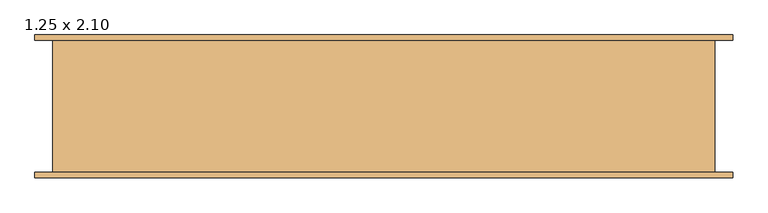
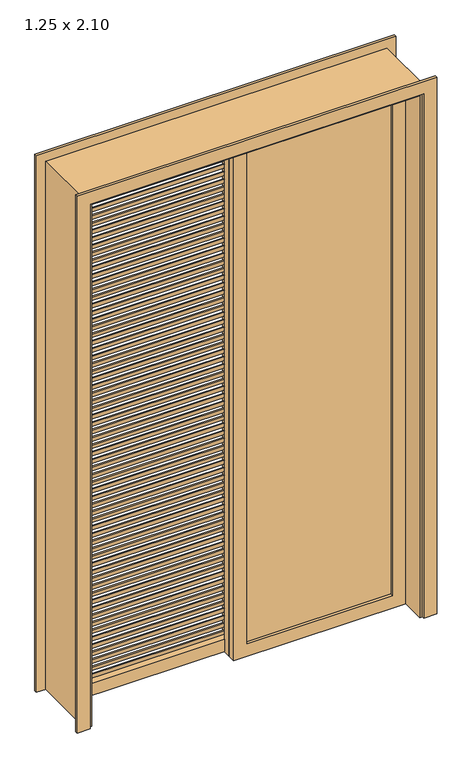
"""IFC4 building model written with IfcOpenShell, lengths in millimetres: door geometry, .CC_ND 300_PORTA DE CORRER_3 FOLHAS_VENEZIANA_VIDRO_COM EXTENSÃO : 1.25 x 2.10."""

from ifc_helpers import new_model, si_unit, frame, origin, place, context, project, spatial, polyline, outline, extrude, source, transform, mapped, element, save


def door_1_25_x_2_10_d20a60c6(model_context):
    return source(origin(), model_context, "Body", "SweptSolid", [
        extrude(outline(polyline([(575.0, -26.0), (575.0, -34.0), (20.0, -34.0), (20.0, -26.0), (575.0, -26.0)])), frame((0.0, 0.0, 50.0), z_axis=(0.0, 0.0, 1.0), x_axis=(1.0, 0.0, 0.0)), (0.0, 0.0, 1.0), 2000.0),
        extrude(outline(polyline([(2100.0, 625.0), (2100.0, -30.0), (0.0, -30.0), (0.0, 625.0), (2100.0, 625.0)]), holes=[polyline([(2050.0, 575.0), (50.0, 575.0), (50.0, 20.0), (2050.0, 20.0), (2050.0, 575.0)])]), frame((0.0, -45.0, 0.0), z_axis=(0.0, 1.0, 0.0), x_axis=(0.0, 0.0, 1.0)), (0.0, 0.0, 1.0), 30.0),
        extrude(outline(polyline([(40.0, 1985.2272727), (15.0, 2020.2272727), (20.0, 2020.2272727), (45.0, 1985.2272727), (40.0, 1985.2272727)])), frame((-575.0, 0.0, 0.0), z_axis=(1.0, 0.0, 0.0), x_axis=(0.0, 1.0, 0.0)), (0.0, 0.0, 1.0), 555.0),
        extrude(outline(polyline([(40.0, 1955.4545455), (15.0, 1990.4545455), (20.0, 1990.4545455), (45.0, 1955.4545455), (40.0, 1955.4545455)])), frame((-575.0, 0.0, 0.0), z_axis=(1.0, 0.0, 0.0), x_axis=(0.0, 1.0, 0.0)), (0.0, 0.0, 1.0), 555.0),
        extrude(outline(polyline([(40.0, 1925.6818182), (15.0, 1960.6818182), (20.0, 1960.6818182), (45.0, 1925.6818182), (40.0, 1925.6818182)])), frame((-575.0, 0.0, 0.0), z_axis=(1.0, 0.0, 0.0), x_axis=(0.0, 1.0, 0.0)), (0.0, 0.0, 1.0), 555.0),
        extrude(outline(polyline([(40.0, 1895.9090909), (15.0, 1930.9090909), (20.0, 1930.9090909), (45.0, 1895.9090909), (40.0, 1895.9090909)])), frame((-575.0, 0.0, 0.0), z_axis=(1.0, 0.0, 0.0), x_axis=(0.0, 1.0, 0.0)), (0.0, 0.0, 1.0), 555.0),
        extrude(outline(polyline([(40.0, 1866.1363636), (15.0, 1901.1363636), (20.0, 1901.1363636), (45.0, 1866.1363636), (40.0, 1866.1363636)])), frame((-575.0, 0.0, 0.0), z_axis=(1.0, 0.0, 0.0), x_axis=(0.0, 1.0, 0.0)), (0.0, 0.0, 1.0), 555.0),
        extrude(outline(polyline([(40.0, 1836.3636364), (15.0, 1871.3636364), (20.0, 1871.3636364), (45.0, 1836.3636364), (40.0, 1836.3636364)])), frame((-575.0, 0.0, 0.0), z_axis=(1.0, 0.0, 0.0), x_axis=(0.0, 1.0, 0.0)), (0.0, 0.0, 1.0), 555.0),
        extrude(outline(polyline([(40.0, 1806.5909091), (15.0, 1841.5909091), (20.0, 1841.5909091), (45.0, 1806.5909091), (40.0, 1806.5909091)])), frame((-575.0, 0.0, 0.0), z_axis=(1.0, 0.0, 0.0), x_axis=(0.0, 1.0, 0.0)), (0.0, 0.0, 1.0), 555.0),
        extrude(outline(polyline([(40.0, 1776.8181818), (15.0, 1811.8181818), (20.0, 1811.8181818), (45.0, 1776.8181818), (40.0, 1776.8181818)])), frame((-575.0, 0.0, 0.0), z_axis=(1.0, 0.0, 0.0), x_axis=(0.0, 1.0, 0.0)), (0.0, 0.0, 1.0), 555.0),
        extrude(outline(polyline([(40.0, 1747.0454545), (15.0, 1782.0454545), (20.0, 1782.0454545), (45.0, 1747.0454545), (40.0, 1747.0454545)])), frame((-575.0, 0.0, 0.0), z_axis=(1.0, 0.0, 0.0), x_axis=(0.0, 1.0, 0.0)), (0.0, 0.0, 1.0), 555.0),
        extrude(outline(polyline([(40.0, 1717.2727273), (15.0, 1752.2727273), (20.0, 1752.2727273), (45.0, 1717.2727273), (40.0, 1717.2727273)])), frame((-575.0, 0.0, 0.0), z_axis=(1.0, 0.0, 0.0), x_axis=(0.0, 1.0, 0.0)), (0.0, 0.0, 1.0), 555.0),
        extrude(outline(polyline([(40.0, 1687.5), (15.0, 1722.5), (20.0, 1722.5), (45.0, 1687.5), (40.0, 1687.5)])), frame((-575.0, 0.0, 0.0), z_axis=(1.0, 0.0, 0.0), x_axis=(0.0, 1.0, 0.0)), (0.0, 0.0, 1.0), 555.0),
        extrude(outline(polyline([(40.0, 1657.7272727), (15.0, 1692.7272727), (20.0, 1692.7272727), (45.0, 1657.7272727), (40.0, 1657.7272727)])), frame((-575.0, 0.0, 0.0), z_axis=(1.0, 0.0, 0.0), x_axis=(0.0, 1.0, 0.0)), (0.0, 0.0, 1.0), 555.0),
        extrude(outline(polyline([(40.0, 1627.9545455), (15.0, 1662.9545455), (20.0, 1662.9545455), (45.0, 1627.9545455), (40.0, 1627.9545455)])), frame((-575.0, 0.0, 0.0), z_axis=(1.0, 0.0, 0.0), x_axis=(0.0, 1.0, 0.0)), (0.0, 0.0, 1.0), 555.0),
        extrude(outline(polyline([(40.0, 1598.1818182), (15.0, 1633.1818182), (20.0, 1633.1818182), (45.0, 1598.1818182), (40.0, 1598.1818182)])), frame((-575.0, 0.0, 0.0), z_axis=(1.0, 0.0, 0.0), x_axis=(0.0, 1.0, 0.0)), (0.0, 0.0, 1.0), 555.0),
        extrude(outline(polyline([(40.0, 1568.4090909), (15.0, 1603.4090909), (20.0, 1603.4090909), (45.0, 1568.4090909), (40.0, 1568.4090909)])), frame((-575.0, 0.0, 0.0), z_axis=(1.0, 0.0, 0.0), x_axis=(0.0, 1.0, 0.0)), (0.0, 0.0, 1.0), 555.0),
        extrude(outline(polyline([(40.0, 1538.6363636), (15.0, 1573.6363636), (20.0, 1573.6363636), (45.0, 1538.6363636), (40.0, 1538.6363636)])), frame((-575.0, 0.0, 0.0), z_axis=(1.0, 0.0, 0.0), x_axis=(0.0, 1.0, 0.0)), (0.0, 0.0, 1.0), 555.0),
        extrude(outline(polyline([(40.0, 1508.8636364), (15.0, 1543.8636364), (20.0, 1543.8636364), (45.0, 1508.8636364), (40.0, 1508.8636364)])), frame((-575.0, 0.0, 0.0), z_axis=(1.0, 0.0, 0.0), x_axis=(0.0, 1.0, 0.0)), (0.0, 0.0, 1.0), 555.0),
        extrude(outline(polyline([(40.0, 1479.0909091), (15.0, 1514.0909091), (20.0, 1514.0909091), (45.0, 1479.0909091), (40.0, 1479.0909091)])), frame((-575.0, 0.0, 0.0), z_axis=(1.0, 0.0, 0.0), x_axis=(0.0, 1.0, 0.0)), (0.0, 0.0, 1.0), 555.0),
        extrude(outline(polyline([(40.0, 1449.3181818), (15.0, 1484.3181818), (20.0, 1484.3181818), (45.0, 1449.3181818), (40.0, 1449.3181818)])), frame((-575.0, 0.0, 0.0), z_axis=(1.0, 0.0, 0.0), x_axis=(0.0, 1.0, 0.0)), (0.0, 0.0, 1.0), 555.0),
        extrude(outline(polyline([(40.0, 1419.5454545), (15.0, 1454.5454545), (20.0, 1454.5454545), (45.0, 1419.5454545), (40.0, 1419.5454545)])), frame((-575.0, 0.0, 0.0), z_axis=(1.0, 0.0, 0.0), x_axis=(0.0, 1.0, 0.0)), (0.0, 0.0, 1.0), 555.0),
        extrude(outline(polyline([(40.0, 1389.7727273), (15.0, 1424.7727273), (20.0, 1424.7727273), (45.0, 1389.7727273), (40.0, 1389.7727273)])), frame((-575.0, 0.0, 0.0), z_axis=(1.0, 0.0, 0.0), x_axis=(0.0, 1.0, 0.0)), (0.0, 0.0, 1.0), 555.0),
        extrude(outline(polyline([(40.0, 1360.0), (15.0, 1395.0), (20.0, 1395.0), (45.0, 1360.0), (40.0, 1360.0)])), frame((-575.0, 0.0, 0.0), z_axis=(1.0, 0.0, 0.0), x_axis=(0.0, 1.0, 0.0)), (0.0, 0.0, 1.0), 555.0),
        extrude(outline(polyline([(40.0, 1330.2272727), (15.0, 1365.2272727), (20.0, 1365.2272727), (45.0, 1330.2272727), (40.0, 1330.2272727)])), frame((-575.0, 0.0, 0.0), z_axis=(1.0, 0.0, 0.0), x_axis=(0.0, 1.0, 0.0)), (0.0, 0.0, 1.0), 555.0),
        extrude(outline(polyline([(40.0, 1300.4545455), (15.0, 1335.4545455), (20.0, 1335.4545455), (45.0, 1300.4545455), (40.0, 1300.4545455)])), frame((-575.0, 0.0, 0.0), z_axis=(1.0, 0.0, 0.0), x_axis=(0.0, 1.0, 0.0)), (0.0, 0.0, 1.0), 555.0),
        extrude(outline(polyline([(40.0, 1270.6818182), (15.0, 1305.6818182), (20.0, 1305.6818182), (45.0, 1270.6818182), (40.0, 1270.6818182)])), frame((-575.0, 0.0, 0.0), z_axis=(1.0, 0.0, 0.0), x_axis=(0.0, 1.0, 0.0)), (0.0, 0.0, 1.0), 555.0),
        extrude(outline(polyline([(40.0, 1240.9090909), (15.0, 1275.9090909), (20.0, 1275.9090909), (45.0, 1240.9090909), (40.0, 1240.9090909)])), frame((-575.0, 0.0, 0.0), z_axis=(1.0, 0.0, 0.0), x_axis=(0.0, 1.0, 0.0)), (0.0, 0.0, 1.0), 555.0),
        extrude(outline(polyline([(40.0, 1211.1363636), (15.0, 1246.1363636), (20.0, 1246.1363636), (45.0, 1211.1363636), (40.0, 1211.1363636)])), frame((-575.0, 0.0, 0.0), z_axis=(1.0, 0.0, 0.0), x_axis=(0.0, 1.0, 0.0)), (0.0, 0.0, 1.0), 555.0),
        extrude(outline(polyline([(40.0, 1181.3636364), (15.0, 1216.3636364), (20.0, 1216.3636364), (45.0, 1181.3636364), (40.0, 1181.3636364)])), frame((-575.0, 0.0, 0.0), z_axis=(1.0, 0.0, 0.0), x_axis=(0.0, 1.0, 0.0)), (0.0, 0.0, 1.0), 555.0),
        extrude(outline(polyline([(40.0, 1151.5909091), (15.0, 1186.5909091), (20.0, 1186.5909091), (45.0, 1151.5909091), (40.0, 1151.5909091)])), frame((-575.0, 0.0, 0.0), z_axis=(1.0, 0.0, 0.0), x_axis=(0.0, 1.0, 0.0)), (0.0, 0.0, 1.0), 555.0),
        extrude(outline(polyline([(40.0, 1121.8181818), (15.0, 1156.8181818), (20.0, 1156.8181818), (45.0, 1121.8181818), (40.0, 1121.8181818)])), frame((-575.0, 0.0, 0.0), z_axis=(1.0, 0.0, 0.0), x_axis=(0.0, 1.0, 0.0)), (0.0, 0.0, 1.0), 555.0),
        extrude(outline(polyline([(40.0, 1092.0454545), (15.0, 1127.0454545), (20.0, 1127.0454545), (45.0, 1092.0454545), (40.0, 1092.0454545)])), frame((-575.0, 0.0, 0.0), z_axis=(1.0, 0.0, 0.0), x_axis=(0.0, 1.0, 0.0)), (0.0, 0.0, 1.0), 555.0),
        extrude(outline(polyline([(40.0, 1062.2727273), (15.0, 1097.2727273), (20.0, 1097.2727273), (45.0, 1062.2727273), (40.0, 1062.2727273)])), frame((-575.0, 0.0, 0.0), z_axis=(1.0, 0.0, 0.0), x_axis=(0.0, 1.0, 0.0)), (0.0, 0.0, 1.0), 555.0),
        extrude(outline(polyline([(40.0, 1032.5), (15.0, 1067.5), (20.0, 1067.5), (45.0, 1032.5), (40.0, 1032.5)])), frame((-575.0, 0.0, 0.0), z_axis=(1.0, 0.0, 0.0), x_axis=(0.0, 1.0, 0.0)), (0.0, 0.0, 1.0), 555.0),
        extrude(outline(polyline([(40.0, 1002.7272727), (15.0, 1037.7272727), (20.0, 1037.7272727), (45.0, 1002.7272727), (40.0, 1002.7272727)])), frame((-575.0, 0.0, 0.0), z_axis=(1.0, 0.0, 0.0), x_axis=(0.0, 1.0, 0.0)), (0.0, 0.0, 1.0), 555.0),
        extrude(outline(polyline([(40.0, 972.9545455), (15.0, 1007.9545455), (20.0, 1007.9545455), (45.0, 972.9545455), (40.0, 972.9545455)])), frame((-575.0, 0.0, 0.0), z_axis=(1.0, 0.0, 0.0), x_axis=(0.0, 1.0, 0.0)), (0.0, 0.0, 1.0), 555.0),
        extrude(outline(polyline([(40.0, 943.1818182), (15.0, 978.1818182), (20.0, 978.1818182), (45.0, 943.1818182), (40.0, 943.1818182)])), frame((-575.0, 0.0, 0.0), z_axis=(1.0, 0.0, 0.0), x_axis=(0.0, 1.0, 0.0)), (0.0, 0.0, 1.0), 555.0),
        extrude(outline(polyline([(40.0, 913.4090909), (15.0, 948.4090909), (20.0, 948.4090909), (45.0, 913.4090909), (40.0, 913.4090909)])), frame((-575.0, 0.0, 0.0), z_axis=(1.0, 0.0, 0.0), x_axis=(0.0, 1.0, 0.0)), (0.0, 0.0, 1.0), 555.0),
        extrude(outline(polyline([(40.0, 883.6363636), (15.0, 918.6363636), (20.0, 918.6363636), (45.0, 883.6363636), (40.0, 883.6363636)])), frame((-575.0, 0.0, 0.0), z_axis=(1.0, 0.0, 0.0), x_axis=(0.0, 1.0, 0.0)), (0.0, 0.0, 1.0), 555.0),
        extrude(outline(polyline([(40.0, 853.8636364), (15.0, 888.8636364), (20.0, 888.8636364), (45.0, 853.8636364), (40.0, 853.8636364)])), frame((-575.0, 0.0, 0.0), z_axis=(1.0, 0.0, 0.0), x_axis=(0.0, 1.0, 0.0)), (0.0, 0.0, 1.0), 555.0),
        extrude(outline(polyline([(40.0, 824.0909091), (15.0, 859.0909091), (20.0, 859.0909091), (45.0, 824.0909091), (40.0, 824.0909091)])), frame((-575.0, 0.0, 0.0), z_axis=(1.0, 0.0, 0.0), x_axis=(0.0, 1.0, 0.0)), (0.0, 0.0, 1.0), 555.0),
        extrude(outline(polyline([(40.0, 794.3181818), (15.0, 829.3181818), (20.0, 829.3181818), (45.0, 794.3181818), (40.0, 794.3181818)])), frame((-575.0, 0.0, 0.0), z_axis=(1.0, 0.0, 0.0), x_axis=(0.0, 1.0, 0.0)), (0.0, 0.0, 1.0), 555.0),
        extrude(outline(polyline([(40.0, 764.5454545), (15.0, 799.5454545), (20.0, 799.5454545), (45.0, 764.5454545), (40.0, 764.5454545)])), frame((-575.0, 0.0, 0.0), z_axis=(1.0, 0.0, 0.0), x_axis=(0.0, 1.0, 0.0)), (0.0, 0.0, 1.0), 555.0),
        extrude(outline(polyline([(40.0, 734.7727273), (15.0, 769.7727273), (20.0, 769.7727273), (45.0, 734.7727273), (40.0, 734.7727273)])), frame((-575.0, 0.0, 0.0), z_axis=(1.0, 0.0, 0.0), x_axis=(0.0, 1.0, 0.0)), (0.0, 0.0, 1.0), 555.0),
        extrude(outline(polyline([(40.0, 705.0), (15.0, 740.0), (20.0, 740.0), (45.0, 705.0), (40.0, 705.0)])), frame((-575.0, 0.0, 0.0), z_axis=(1.0, 0.0, 0.0), x_axis=(0.0, 1.0, 0.0)), (0.0, 0.0, 1.0), 555.0),
        extrude(outline(polyline([(40.0, 675.2272727), (15.0, 710.2272727), (20.0, 710.2272727), (45.0, 675.2272727), (40.0, 675.2272727)])), frame((-575.0, 0.0, 0.0), z_axis=(1.0, 0.0, 0.0), x_axis=(0.0, 1.0, 0.0)), (0.0, 0.0, 1.0), 555.0),
        extrude(outline(polyline([(40.0, 645.4545455), (15.0, 680.4545455), (20.0, 680.4545455), (45.0, 645.4545455), (40.0, 645.4545455)])), frame((-575.0, 0.0, 0.0), z_axis=(1.0, 0.0, 0.0), x_axis=(0.0, 1.0, 0.0)), (0.0, 0.0, 1.0), 555.0),
        extrude(outline(polyline([(40.0, 615.6818182), (15.0, 650.6818182), (20.0, 650.6818182), (45.0, 615.6818182), (40.0, 615.6818182)])), frame((-575.0, 0.0, 0.0), z_axis=(1.0, 0.0, 0.0), x_axis=(0.0, 1.0, 0.0)), (0.0, 0.0, 1.0), 555.0),
        extrude(outline(polyline([(40.0, 585.9090909), (15.0, 620.9090909), (20.0, 620.9090909), (45.0, 585.9090909), (40.0, 585.9090909)])), frame((-575.0, 0.0, 0.0), z_axis=(1.0, 0.0, 0.0), x_axis=(0.0, 1.0, 0.0)), (0.0, 0.0, 1.0), 555.0),
        extrude(outline(polyline([(40.0, 556.1363636), (15.0, 591.1363636), (20.0, 591.1363636), (45.0, 556.1363636), (40.0, 556.1363636)])), frame((-575.0, 0.0, 0.0), z_axis=(1.0, 0.0, 0.0), x_axis=(0.0, 1.0, 0.0)), (0.0, 0.0, 1.0), 555.0),
        extrude(outline(polyline([(40.0, 526.3636364), (15.0, 561.3636364), (20.0, 561.3636364), (45.0, 526.3636364), (40.0, 526.3636364)])), frame((-575.0, 0.0, 0.0), z_axis=(1.0, 0.0, 0.0), x_axis=(0.0, 1.0, 0.0)), (0.0, 0.0, 1.0), 555.0),
        extrude(outline(polyline([(40.0, 496.5909091), (15.0, 531.5909091), (20.0, 531.5909091), (45.0, 496.5909091), (40.0, 496.5909091)])), frame((-575.0, 0.0, 0.0), z_axis=(1.0, 0.0, 0.0), x_axis=(0.0, 1.0, 0.0)), (0.0, 0.0, 1.0), 555.0),
        extrude(outline(polyline([(40.0, 466.8181818), (15.0, 501.8181818), (20.0, 501.8181818), (45.0, 466.8181818), (40.0, 466.8181818)])), frame((-575.0, 0.0, 0.0), z_axis=(1.0, 0.0, 0.0), x_axis=(0.0, 1.0, 0.0)), (0.0, 0.0, 1.0), 555.0),
        extrude(outline(polyline([(40.0, 437.0454545), (15.0, 472.0454545), (20.0, 472.0454545), (45.0, 437.0454545), (40.0, 437.0454545)])), frame((-575.0, 0.0, 0.0), z_axis=(1.0, 0.0, 0.0), x_axis=(0.0, 1.0, 0.0)), (0.0, 0.0, 1.0), 555.0),
        extrude(outline(polyline([(40.0, 407.2727273), (15.0, 442.2727273), (20.0, 442.2727273), (45.0, 407.2727273), (40.0, 407.2727273)])), frame((-575.0, 0.0, 0.0), z_axis=(1.0, 0.0, 0.0), x_axis=(0.0, 1.0, 0.0)), (0.0, 0.0, 1.0), 555.0),
        extrude(outline(polyline([(40.0, 377.5), (15.0, 412.5), (20.0, 412.5), (45.0, 377.5), (40.0, 377.5)])), frame((-575.0, 0.0, 0.0), z_axis=(1.0, 0.0, 0.0), x_axis=(0.0, 1.0, 0.0)), (0.0, 0.0, 1.0), 555.0),
        extrude(outline(polyline([(40.0, 347.7272727), (15.0, 382.7272727), (20.0, 382.7272727), (45.0, 347.7272727), (40.0, 347.7272727)])), frame((-575.0, 0.0, 0.0), z_axis=(1.0, 0.0, 0.0), x_axis=(0.0, 1.0, 0.0)), (0.0, 0.0, 1.0), 555.0),
        extrude(outline(polyline([(40.0, 317.9545455), (15.0, 352.9545455), (20.0, 352.9545455), (45.0, 317.9545455), (40.0, 317.9545455)])), frame((-575.0, 0.0, 0.0), z_axis=(1.0, 0.0, 0.0), x_axis=(0.0, 1.0, 0.0)), (0.0, 0.0, 1.0), 555.0),
        extrude(outline(polyline([(40.0, 288.1818182), (15.0, 323.1818182), (20.0, 323.1818182), (45.0, 288.1818182), (40.0, 288.1818182)])), frame((-575.0, 0.0, 0.0), z_axis=(1.0, 0.0, 0.0), x_axis=(0.0, 1.0, 0.0)), (0.0, 0.0, 1.0), 555.0),
        extrude(outline(polyline([(40.0, 258.4090909), (15.0, 293.4090909), (20.0, 293.4090909), (45.0, 258.4090909), (40.0, 258.4090909)])), frame((-575.0, 0.0, 0.0), z_axis=(1.0, 0.0, 0.0), x_axis=(0.0, 1.0, 0.0)), (0.0, 0.0, 1.0), 555.0),
        extrude(outline(polyline([(40.0, 228.6363636), (15.0, 263.6363636), (20.0, 263.6363636), (45.0, 228.6363636), (40.0, 228.6363636)])), frame((-575.0, 0.0, 0.0), z_axis=(1.0, 0.0, 0.0), x_axis=(0.0, 1.0, 0.0)), (0.0, 0.0, 1.0), 555.0),
        extrude(outline(polyline([(40.0, 198.8636364), (15.0, 233.8636364), (20.0, 233.8636364), (45.0, 198.8636364), (40.0, 198.8636364)])), frame((-575.0, 0.0, 0.0), z_axis=(1.0, 0.0, 0.0), x_axis=(0.0, 1.0, 0.0)), (0.0, 0.0, 1.0), 555.0),
        extrude(outline(polyline([(40.0, 169.0909091), (15.0, 204.0909091), (20.0, 204.0909091), (45.0, 169.0909091), (40.0, 169.0909091)])), frame((-575.0, 0.0, 0.0), z_axis=(1.0, 0.0, 0.0), x_axis=(0.0, 1.0, 0.0)), (0.0, 0.0, 1.0), 555.0),
        extrude(outline(polyline([(40.0, 139.3181818), (15.0, 174.3181818), (20.0, 174.3181818), (45.0, 139.3181818), (40.0, 139.3181818)])), frame((-575.0, 0.0, 0.0), z_axis=(1.0, 0.0, 0.0), x_axis=(0.0, 1.0, 0.0)), (0.0, 0.0, 1.0), 555.0),
        extrude(outline(polyline([(40.0, 109.5454545), (15.0, 144.5454545), (20.0, 144.5454545), (45.0, 109.5454545), (40.0, 109.5454545)])), frame((-575.0, 0.0, 0.0), z_axis=(1.0, 0.0, 0.0), x_axis=(0.0, 1.0, 0.0)), (0.0, 0.0, 1.0), 555.0),
        extrude(outline(polyline([(40.0, 79.7727273), (15.0, 114.7727273), (20.0, 114.7727273), (45.0, 79.7727273), (40.0, 79.7727273)])), frame((-575.0, 0.0, 0.0), z_axis=(1.0, 0.0, 0.0), x_axis=(0.0, 1.0, 0.0)), (0.0, 0.0, 1.0), 555.0),
        extrude(outline(polyline([(40.0, 2015.0), (15.0, 2050.0), (20.0, 2050.0), (45.0, 2015.0), (40.0, 2015.0)])), frame((-575.0, 0.0, 0.0), z_axis=(1.0, 0.0, 0.0), x_axis=(0.0, 1.0, 0.0)), (0.0, 0.0, 1.0), 555.0),
        extrude(outline(polyline([(40.0, 50.0), (15.0, 85.0), (20.0, 85.0), (45.0, 50.0), (40.0, 50.0)])), frame((-575.0, 0.0, 0.0), z_axis=(1.0, 0.0, 0.0), x_axis=(0.0, 1.0, 0.0)), (0.0, 0.0, 1.0), 555.0),
        extrude(outline(polyline([(2100.0, 30.0), (2100.0, -625.0), (0.0, -625.0), (0.0, 30.0), (2100.0, 30.0)]), holes=[polyline([(2050.0, -20.0), (50.0, -20.0), (50.0, -575.0), (2050.0, -575.0), (2050.0, -20.0)])]), frame((0.0, 15.0, 0.0), z_axis=(0.0, 1.0, 0.0), x_axis=(0.0, 0.0, 1.0)), (0.0, 0.0, 1.0), 30.0),
        extrude(outline(polyline([(10.0, 1985.2272727), (-15.0, 2020.2272727), (-10.0, 2020.2272727), (15.0, 1985.2272727), (10.0, 1985.2272727)])), frame((20.0, 0.0, 0.0), z_axis=(1.0, 0.0, 0.0), x_axis=(0.0, 1.0, 0.0)), (0.0, 0.0, 1.0), 555.0),
        extrude(outline(polyline([(10.0, 1955.4545455), (-15.0, 1990.4545455), (-10.0, 1990.4545455), (15.0, 1955.4545455), (10.0, 1955.4545455)])), frame((20.0, 0.0, 0.0), z_axis=(1.0, 0.0, 0.0), x_axis=(0.0, 1.0, 0.0)), (0.0, 0.0, 1.0), 555.0),
        extrude(outline(polyline([(10.0, 1925.6818182), (-15.0, 1960.6818182), (-10.0, 1960.6818182), (15.0, 1925.6818182), (10.0, 1925.6818182)])), frame((20.0, 0.0, 0.0), z_axis=(1.0, 0.0, 0.0), x_axis=(0.0, 1.0, 0.0)), (0.0, 0.0, 1.0), 555.0),
        extrude(outline(polyline([(10.0, 1895.9090909), (-15.0, 1930.9090909), (-10.0, 1930.9090909), (15.0, 1895.9090909), (10.0, 1895.9090909)])), frame((20.0, 0.0, 0.0), z_axis=(1.0, 0.0, 0.0), x_axis=(0.0, 1.0, 0.0)), (0.0, 0.0, 1.0), 555.0),
        extrude(outline(polyline([(10.0, 1866.1363636), (-15.0, 1901.1363636), (-10.0, 1901.1363636), (15.0, 1866.1363636), (10.0, 1866.1363636)])), frame((20.0, 0.0, 0.0), z_axis=(1.0, 0.0, 0.0), x_axis=(0.0, 1.0, 0.0)), (0.0, 0.0, 1.0), 555.0),
        extrude(outline(polyline([(10.0, 1836.3636364), (-15.0, 1871.3636364), (-10.0, 1871.3636364), (15.0, 1836.3636364), (10.0, 1836.3636364)])), frame((20.0, 0.0, 0.0), z_axis=(1.0, 0.0, 0.0), x_axis=(0.0, 1.0, 0.0)), (0.0, 0.0, 1.0), 555.0),
        extrude(outline(polyline([(10.0, 1806.5909091), (-15.0, 1841.5909091), (-10.0, 1841.5909091), (15.0, 1806.5909091), (10.0, 1806.5909091)])), frame((20.0, 0.0, 0.0), z_axis=(1.0, 0.0, 0.0), x_axis=(0.0, 1.0, 0.0)), (0.0, 0.0, 1.0), 555.0),
        extrude(outline(polyline([(10.0, 1776.8181818), (-15.0, 1811.8181818), (-10.0, 1811.8181818), (15.0, 1776.8181818), (10.0, 1776.8181818)])), frame((20.0, 0.0, 0.0), z_axis=(1.0, 0.0, 0.0), x_axis=(0.0, 1.0, 0.0)), (0.0, 0.0, 1.0), 555.0),
        extrude(outline(polyline([(10.0, 1747.0454545), (-15.0, 1782.0454545), (-10.0, 1782.0454545), (15.0, 1747.0454545), (10.0, 1747.0454545)])), frame((20.0, 0.0, 0.0), z_axis=(1.0, 0.0, 0.0), x_axis=(0.0, 1.0, 0.0)), (0.0, 0.0, 1.0), 555.0),
        extrude(outline(polyline([(10.0, 1717.2727273), (-15.0, 1752.2727273), (-10.0, 1752.2727273), (15.0, 1717.2727273), (10.0, 1717.2727273)])), frame((20.0, 0.0, 0.0), z_axis=(1.0, 0.0, 0.0), x_axis=(0.0, 1.0, 0.0)), (0.0, 0.0, 1.0), 555.0),
        extrude(outline(polyline([(10.0, 1687.5), (-15.0, 1722.5), (-10.0, 1722.5), (15.0, 1687.5), (10.0, 1687.5)])), frame((20.0, 0.0, 0.0), z_axis=(1.0, 0.0, 0.0), x_axis=(0.0, 1.0, 0.0)), (0.0, 0.0, 1.0), 555.0),
        extrude(outline(polyline([(10.0, 1657.7272727), (-15.0, 1692.7272727), (-10.0, 1692.7272727), (15.0, 1657.7272727), (10.0, 1657.7272727)])), frame((20.0, 0.0, 0.0), z_axis=(1.0, 0.0, 0.0), x_axis=(0.0, 1.0, 0.0)), (0.0, 0.0, 1.0), 555.0),
        extrude(outline(polyline([(10.0, 1627.9545455), (-15.0, 1662.9545455), (-10.0, 1662.9545455), (15.0, 1627.9545455), (10.0, 1627.9545455)])), frame((20.0, 0.0, 0.0), z_axis=(1.0, 0.0, 0.0), x_axis=(0.0, 1.0, 0.0)), (0.0, 0.0, 1.0), 555.0),
        extrude(outline(polyline([(10.0, 1598.1818182), (-15.0, 1633.1818182), (-10.0, 1633.1818182), (15.0, 1598.1818182), (10.0, 1598.1818182)])), frame((20.0, 0.0, 0.0), z_axis=(1.0, 0.0, 0.0), x_axis=(0.0, 1.0, 0.0)), (0.0, 0.0, 1.0), 555.0),
        extrude(outline(polyline([(10.0, 1568.4090909), (-15.0, 1603.4090909), (-10.0, 1603.4090909), (15.0, 1568.4090909), (10.0, 1568.4090909)])), frame((20.0, 0.0, 0.0), z_axis=(1.0, 0.0, 0.0), x_axis=(0.0, 1.0, 0.0)), (0.0, 0.0, 1.0), 555.0),
        extrude(outline(polyline([(10.0, 1538.6363636), (-15.0, 1573.6363636), (-10.0, 1573.6363636), (15.0, 1538.6363636), (10.0, 1538.6363636)])), frame((20.0, 0.0, 0.0), z_axis=(1.0, 0.0, 0.0), x_axis=(0.0, 1.0, 0.0)), (0.0, 0.0, 1.0), 555.0),
        extrude(outline(polyline([(10.0, 1508.8636364), (-15.0, 1543.8636364), (-10.0, 1543.8636364), (15.0, 1508.8636364), (10.0, 1508.8636364)])), frame((20.0, 0.0, 0.0), z_axis=(1.0, 0.0, 0.0), x_axis=(0.0, 1.0, 0.0)), (0.0, 0.0, 1.0), 555.0),
        extrude(outline(polyline([(10.0, 1479.0909091), (-15.0, 1514.0909091), (-10.0, 1514.0909091), (15.0, 1479.0909091), (10.0, 1479.0909091)])), frame((20.0, 0.0, 0.0), z_axis=(1.0, 0.0, 0.0), x_axis=(0.0, 1.0, 0.0)), (0.0, 0.0, 1.0), 555.0),
        extrude(outline(polyline([(10.0, 1449.3181818), (-15.0, 1484.3181818), (-10.0, 1484.3181818), (15.0, 1449.3181818), (10.0, 1449.3181818)])), frame((20.0, 0.0, 0.0), z_axis=(1.0, 0.0, 0.0), x_axis=(0.0, 1.0, 0.0)), (0.0, 0.0, 1.0), 555.0),
        extrude(outline(polyline([(10.0, 1419.5454545), (-15.0, 1454.5454545), (-10.0, 1454.5454545), (15.0, 1419.5454545), (10.0, 1419.5454545)])), frame((20.0, 0.0, 0.0), z_axis=(1.0, 0.0, 0.0), x_axis=(0.0, 1.0, 0.0)), (0.0, 0.0, 1.0), 555.0),
        extrude(outline(polyline([(10.0, 1389.7727273), (-15.0, 1424.7727273), (-10.0, 1424.7727273), (15.0, 1389.7727273), (10.0, 1389.7727273)])), frame((20.0, 0.0, 0.0), z_axis=(1.0, 0.0, 0.0), x_axis=(0.0, 1.0, 0.0)), (0.0, 0.0, 1.0), 555.0),
        extrude(outline(polyline([(10.0, 1360.0), (-15.0, 1395.0), (-10.0, 1395.0), (15.0, 1360.0), (10.0, 1360.0)])), frame((20.0, 0.0, 0.0), z_axis=(1.0, 0.0, 0.0), x_axis=(0.0, 1.0, 0.0)), (0.0, 0.0, 1.0), 555.0),
        extrude(outline(polyline([(10.0, 1330.2272727), (-15.0, 1365.2272727), (-10.0, 1365.2272727), (15.0, 1330.2272727), (10.0, 1330.2272727)])), frame((20.0, 0.0, 0.0), z_axis=(1.0, 0.0, 0.0), x_axis=(0.0, 1.0, 0.0)), (0.0, 0.0, 1.0), 555.0),
        extrude(outline(polyline([(10.0, 1300.4545455), (-15.0, 1335.4545455), (-10.0, 1335.4545455), (15.0, 1300.4545455), (10.0, 1300.4545455)])), frame((20.0, 0.0, 0.0), z_axis=(1.0, 0.0, 0.0), x_axis=(0.0, 1.0, 0.0)), (0.0, 0.0, 1.0), 555.0),
        extrude(outline(polyline([(10.0, 1270.6818182), (-15.0, 1305.6818182), (-10.0, 1305.6818182), (15.0, 1270.6818182), (10.0, 1270.6818182)])), frame((20.0, 0.0, 0.0), z_axis=(1.0, 0.0, 0.0), x_axis=(0.0, 1.0, 0.0)), (0.0, 0.0, 1.0), 555.0),
        extrude(outline(polyline([(10.0, 1240.9090909), (-15.0, 1275.9090909), (-10.0, 1275.9090909), (15.0, 1240.9090909), (10.0, 1240.9090909)])), frame((20.0, 0.0, 0.0), z_axis=(1.0, 0.0, 0.0), x_axis=(0.0, 1.0, 0.0)), (0.0, 0.0, 1.0), 555.0),
        extrude(outline(polyline([(10.0, 1211.1363636), (-15.0, 1246.1363636), (-10.0, 1246.1363636), (15.0, 1211.1363636), (10.0, 1211.1363636)])), frame((20.0, 0.0, 0.0), z_axis=(1.0, 0.0, 0.0), x_axis=(0.0, 1.0, 0.0)), (0.0, 0.0, 1.0), 555.0),
        extrude(outline(polyline([(10.0, 1181.3636364), (-15.0, 1216.3636364), (-10.0, 1216.3636364), (15.0, 1181.3636364), (10.0, 1181.3636364)])), frame((20.0, 0.0, 0.0), z_axis=(1.0, 0.0, 0.0), x_axis=(0.0, 1.0, 0.0)), (0.0, 0.0, 1.0), 555.0),
        extrude(outline(polyline([(10.0, 1151.5909091), (-15.0, 1186.5909091), (-10.0, 1186.5909091), (15.0, 1151.5909091), (10.0, 1151.5909091)])), frame((20.0, 0.0, 0.0), z_axis=(1.0, 0.0, 0.0), x_axis=(0.0, 1.0, 0.0)), (0.0, 0.0, 1.0), 555.0),
        extrude(outline(polyline([(10.0, 1121.8181818), (-15.0, 1156.8181818), (-10.0, 1156.8181818), (15.0, 1121.8181818), (10.0, 1121.8181818)])), frame((20.0, 0.0, 0.0), z_axis=(1.0, 0.0, 0.0), x_axis=(0.0, 1.0, 0.0)), (0.0, 0.0, 1.0), 555.0),
        extrude(outline(polyline([(10.0, 1092.0454545), (-15.0, 1127.0454545), (-10.0, 1127.0454545), (15.0, 1092.0454545), (10.0, 1092.0454545)])), frame((20.0, 0.0, 0.0), z_axis=(1.0, 0.0, 0.0), x_axis=(0.0, 1.0, 0.0)), (0.0, 0.0, 1.0), 555.0),
        extrude(outline(polyline([(10.0, 1062.2727273), (-15.0, 1097.2727273), (-10.0, 1097.2727273), (15.0, 1062.2727273), (10.0, 1062.2727273)])), frame((20.0, 0.0, 0.0), z_axis=(1.0, 0.0, 0.0), x_axis=(0.0, 1.0, 0.0)), (0.0, 0.0, 1.0), 555.0),
        extrude(outline(polyline([(10.0, 1032.5), (-15.0, 1067.5), (-10.0, 1067.5), (15.0, 1032.5), (10.0, 1032.5)])), frame((20.0, 0.0, 0.0), z_axis=(1.0, 0.0, 0.0), x_axis=(0.0, 1.0, 0.0)), (0.0, 0.0, 1.0), 555.0),
        extrude(outline(polyline([(10.0, 1002.7272727), (-15.0, 1037.7272727), (-10.0, 1037.7272727), (15.0, 1002.7272727), (10.0, 1002.7272727)])), frame((20.0, 0.0, 0.0), z_axis=(1.0, 0.0, 0.0), x_axis=(0.0, 1.0, 0.0)), (0.0, 0.0, 1.0), 555.0),
        extrude(outline(polyline([(10.0, 972.9545455), (-15.0, 1007.9545455), (-10.0, 1007.9545455), (15.0, 972.9545455), (10.0, 972.9545455)])), frame((20.0, 0.0, 0.0), z_axis=(1.0, 0.0, 0.0), x_axis=(0.0, 1.0, 0.0)), (0.0, 0.0, 1.0), 555.0),
        extrude(outline(polyline([(10.0, 943.1818182), (-15.0, 978.1818182), (-10.0, 978.1818182), (15.0, 943.1818182), (10.0, 943.1818182)])), frame((20.0, 0.0, 0.0), z_axis=(1.0, 0.0, 0.0), x_axis=(0.0, 1.0, 0.0)), (0.0, 0.0, 1.0), 555.0),
        extrude(outline(polyline([(10.0, 913.4090909), (-15.0, 948.4090909), (-10.0, 948.4090909), (15.0, 913.4090909), (10.0, 913.4090909)])), frame((20.0, 0.0, 0.0), z_axis=(1.0, 0.0, 0.0), x_axis=(0.0, 1.0, 0.0)), (0.0, 0.0, 1.0), 555.0),
        extrude(outline(polyline([(10.0, 883.6363636), (-15.0, 918.6363636), (-10.0, 918.6363636), (15.0, 883.6363636), (10.0, 883.6363636)])), frame((20.0, 0.0, 0.0), z_axis=(1.0, 0.0, 0.0), x_axis=(0.0, 1.0, 0.0)), (0.0, 0.0, 1.0), 555.0),
        extrude(outline(polyline([(10.0, 853.8636364), (-15.0, 888.8636364), (-10.0, 888.8636364), (15.0, 853.8636364), (10.0, 853.8636364)])), frame((20.0, 0.0, 0.0), z_axis=(1.0, 0.0, 0.0), x_axis=(0.0, 1.0, 0.0)), (0.0, 0.0, 1.0), 555.0),
        extrude(outline(polyline([(10.0, 824.0909091), (-15.0, 859.0909091), (-10.0, 859.0909091), (15.0, 824.0909091), (10.0, 824.0909091)])), frame((20.0, 0.0, 0.0), z_axis=(1.0, 0.0, 0.0), x_axis=(0.0, 1.0, 0.0)), (0.0, 0.0, 1.0), 555.0),
        extrude(outline(polyline([(10.0, 794.3181818), (-15.0, 829.3181818), (-10.0, 829.3181818), (15.0, 794.3181818), (10.0, 794.3181818)])), frame((20.0, 0.0, 0.0), z_axis=(1.0, 0.0, 0.0), x_axis=(0.0, 1.0, 0.0)), (0.0, 0.0, 1.0), 555.0),
        extrude(outline(polyline([(10.0, 764.5454545), (-15.0, 799.5454545), (-10.0, 799.5454545), (15.0, 764.5454545), (10.0, 764.5454545)])), frame((20.0, 0.0, 0.0), z_axis=(1.0, 0.0, 0.0), x_axis=(0.0, 1.0, 0.0)), (0.0, 0.0, 1.0), 555.0),
        extrude(outline(polyline([(10.0, 734.7727273), (-15.0, 769.7727273), (-10.0, 769.7727273), (15.0, 734.7727273), (10.0, 734.7727273)])), frame((20.0, 0.0, 0.0), z_axis=(1.0, 0.0, 0.0), x_axis=(0.0, 1.0, 0.0)), (0.0, 0.0, 1.0), 555.0),
        extrude(outline(polyline([(10.0, 705.0), (-15.0, 740.0), (-10.0, 740.0), (15.0, 705.0), (10.0, 705.0)])), frame((20.0, 0.0, 0.0), z_axis=(1.0, 0.0, 0.0), x_axis=(0.0, 1.0, 0.0)), (0.0, 0.0, 1.0), 555.0),
        extrude(outline(polyline([(10.0, 675.2272727), (-15.0, 710.2272727), (-10.0, 710.2272727), (15.0, 675.2272727), (10.0, 675.2272727)])), frame((20.0, 0.0, 0.0), z_axis=(1.0, 0.0, 0.0), x_axis=(0.0, 1.0, 0.0)), (0.0, 0.0, 1.0), 555.0),
        extrude(outline(polyline([(10.0, 645.4545455), (-15.0, 680.4545455), (-10.0, 680.4545455), (15.0, 645.4545455), (10.0, 645.4545455)])), frame((20.0, 0.0, 0.0), z_axis=(1.0, 0.0, 0.0), x_axis=(0.0, 1.0, 0.0)), (0.0, 0.0, 1.0), 555.0),
        extrude(outline(polyline([(10.0, 615.6818182), (-15.0, 650.6818182), (-10.0, 650.6818182), (15.0, 615.6818182), (10.0, 615.6818182)])), frame((20.0, 0.0, 0.0), z_axis=(1.0, 0.0, 0.0), x_axis=(0.0, 1.0, 0.0)), (0.0, 0.0, 1.0), 555.0),
        extrude(outline(polyline([(10.0, 585.9090909), (-15.0, 620.9090909), (-10.0, 620.9090909), (15.0, 585.9090909), (10.0, 585.9090909)])), frame((20.0, 0.0, 0.0), z_axis=(1.0, 0.0, 0.0), x_axis=(0.0, 1.0, 0.0)), (0.0, 0.0, 1.0), 555.0),
        extrude(outline(polyline([(10.0, 556.1363636), (-15.0, 591.1363636), (-10.0, 591.1363636), (15.0, 556.1363636), (10.0, 556.1363636)])), frame((20.0, 0.0, 0.0), z_axis=(1.0, 0.0, 0.0), x_axis=(0.0, 1.0, 0.0)), (0.0, 0.0, 1.0), 555.0),
        extrude(outline(polyline([(10.0, 526.3636364), (-15.0, 561.3636364), (-10.0, 561.3636364), (15.0, 526.3636364), (10.0, 526.3636364)])), frame((20.0, 0.0, 0.0), z_axis=(1.0, 0.0, 0.0), x_axis=(0.0, 1.0, 0.0)), (0.0, 0.0, 1.0), 555.0),
        extrude(outline(polyline([(10.0, 496.5909091), (-15.0, 531.5909091), (-10.0, 531.5909091), (15.0, 496.5909091), (10.0, 496.5909091)])), frame((20.0, 0.0, 0.0), z_axis=(1.0, 0.0, 0.0), x_axis=(0.0, 1.0, 0.0)), (0.0, 0.0, 1.0), 555.0),
        extrude(outline(polyline([(10.0, 466.8181818), (-15.0, 501.8181818), (-10.0, 501.8181818), (15.0, 466.8181818), (10.0, 466.8181818)])), frame((20.0, 0.0, 0.0), z_axis=(1.0, 0.0, 0.0), x_axis=(0.0, 1.0, 0.0)), (0.0, 0.0, 1.0), 555.0),
        extrude(outline(polyline([(10.0, 437.0454545), (-15.0, 472.0454545), (-10.0, 472.0454545), (15.0, 437.0454545), (10.0, 437.0454545)])), frame((20.0, 0.0, 0.0), z_axis=(1.0, 0.0, 0.0), x_axis=(0.0, 1.0, 0.0)), (0.0, 0.0, 1.0), 555.0),
        extrude(outline(polyline([(10.0, 407.2727273), (-15.0, 442.2727273), (-10.0, 442.2727273), (15.0, 407.2727273), (10.0, 407.2727273)])), frame((20.0, 0.0, 0.0), z_axis=(1.0, 0.0, 0.0), x_axis=(0.0, 1.0, 0.0)), (0.0, 0.0, 1.0), 555.0),
        extrude(outline(polyline([(10.0, 377.5), (-15.0, 412.5), (-10.0, 412.5), (15.0, 377.5), (10.0, 377.5)])), frame((20.0, 0.0, 0.0), z_axis=(1.0, 0.0, 0.0), x_axis=(0.0, 1.0, 0.0)), (0.0, 0.0, 1.0), 555.0),
        extrude(outline(polyline([(10.0, 347.7272727), (-15.0, 382.7272727), (-10.0, 382.7272727), (15.0, 347.7272727), (10.0, 347.7272727)])), frame((20.0, 0.0, 0.0), z_axis=(1.0, 0.0, 0.0), x_axis=(0.0, 1.0, 0.0)), (0.0, 0.0, 1.0), 555.0),
        extrude(outline(polyline([(10.0, 317.9545455), (-15.0, 352.9545455), (-10.0, 352.9545455), (15.0, 317.9545455), (10.0, 317.9545455)])), frame((20.0, 0.0, 0.0), z_axis=(1.0, 0.0, 0.0), x_axis=(0.0, 1.0, 0.0)), (0.0, 0.0, 1.0), 555.0),
        extrude(outline(polyline([(10.0, 288.1818182), (-15.0, 323.1818182), (-10.0, 323.1818182), (15.0, 288.1818182), (10.0, 288.1818182)])), frame((20.0, 0.0, 0.0), z_axis=(1.0, 0.0, 0.0), x_axis=(0.0, 1.0, 0.0)), (0.0, 0.0, 1.0), 555.0),
        extrude(outline(polyline([(10.0, 258.4090909), (-15.0, 293.4090909), (-10.0, 293.4090909), (15.0, 258.4090909), (10.0, 258.4090909)])), frame((20.0, 0.0, 0.0), z_axis=(1.0, 0.0, 0.0), x_axis=(0.0, 1.0, 0.0)), (0.0, 0.0, 1.0), 555.0),
        extrude(outline(polyline([(10.0, 228.6363636), (-15.0, 263.6363636), (-10.0, 263.6363636), (15.0, 228.6363636), (10.0, 228.6363636)])), frame((20.0, 0.0, 0.0), z_axis=(1.0, 0.0, 0.0), x_axis=(0.0, 1.0, 0.0)), (0.0, 0.0, 1.0), 555.0),
        extrude(outline(polyline([(10.0, 198.8636364), (-15.0, 233.8636364), (-10.0, 233.8636364), (15.0, 198.8636364), (10.0, 198.8636364)])), frame((20.0, 0.0, 0.0), z_axis=(1.0, 0.0, 0.0), x_axis=(0.0, 1.0, 0.0)), (0.0, 0.0, 1.0), 555.0),
        extrude(outline(polyline([(10.0, 169.0909091), (-15.0, 204.0909091), (-10.0, 204.0909091), (15.0, 169.0909091), (10.0, 169.0909091)])), frame((20.0, 0.0, 0.0), z_axis=(1.0, 0.0, 0.0), x_axis=(0.0, 1.0, 0.0)), (0.0, 0.0, 1.0), 555.0),
        extrude(outline(polyline([(10.0, 139.3181818), (-15.0, 174.3181818), (-10.0, 174.3181818), (15.0, 139.3181818), (10.0, 139.3181818)])), frame((20.0, 0.0, 0.0), z_axis=(1.0, 0.0, 0.0), x_axis=(0.0, 1.0, 0.0)), (0.0, 0.0, 1.0), 555.0),
        extrude(outline(polyline([(10.0, 109.5454545), (-15.0, 144.5454545), (-10.0, 144.5454545), (15.0, 109.5454545), (10.0, 109.5454545)])), frame((20.0, 0.0, 0.0), z_axis=(1.0, 0.0, 0.0), x_axis=(0.0, 1.0, 0.0)), (0.0, 0.0, 1.0), 555.0),
        extrude(outline(polyline([(10.0, 79.7727273), (-15.0, 114.7727273), (-10.0, 114.7727273), (15.0, 79.7727273), (10.0, 79.7727273)])), frame((20.0, 0.0, 0.0), z_axis=(1.0, 0.0, 0.0), x_axis=(0.0, 1.0, 0.0)), (0.0, 0.0, 1.0), 555.0),
        extrude(outline(polyline([(10.0, 2015.0), (-15.0, 2050.0), (-10.0, 2050.0), (15.0, 2015.0), (10.0, 2015.0)])), frame((20.0, 0.0, 0.0), z_axis=(1.0, 0.0, 0.0), x_axis=(0.0, 1.0, 0.0)), (0.0, 0.0, 1.0), 555.0),
        extrude(outline(polyline([(10.0, 50.0), (-15.0, 85.0), (-10.0, 85.0), (15.0, 50.0), (10.0, 50.0)])), frame((20.0, 0.0, 0.0), z_axis=(1.0, 0.0, 0.0), x_axis=(0.0, 1.0, 0.0)), (0.0, 0.0, 1.0), 555.0),
        extrude(outline(polyline([(2100.0, 625.0), (2100.0, -30.0), (0.0, -30.0), (0.0, 625.0), (2100.0, 625.0)]), holes=[polyline([(2050.0, 575.0), (50.0, 575.0), (50.0, 20.0), (2050.0, 20.0), (2050.0, 575.0)])]), frame((0.0, -15.0, 0.0), z_axis=(0.0, 1.0, 0.0), x_axis=(0.0, 0.0, 1.0)), (0.0, 0.0, 1.0), 30.0),
        extrude(outline(polyline([(0.0, 635.0), (0.0, 685.0), (2160.0, 685.0), (2160.0, -685.0), (0.0, -685.0), (0.0, -635.0), (2110.0, -635.0), (2110.0, 635.0), (0.0, 635.0)])), frame((0.0, 122.4, 0.0), z_axis=(0.0, 1.0, 0.0), x_axis=(0.0, 0.0, 1.0)), (0.0, 0.0, 1.0), 10.0),
        extrude(outline(polyline([(0.0, -685.0), (0.0, -635.0), (2110.0, -635.0), (2110.0, 635.0), (0.0, 635.0), (0.0, 685.0), (2160.0, 685.0), (2160.0, -685.0), (0.0, -685.0)])), frame((0.0, -147.4, 0.0), z_axis=(0.0, 1.0, 0.0), x_axis=(0.0, 0.0, 1.0)), (0.0, 0.0, 1.0), 10.0),
        extrude(outline(polyline([(0.0, -650.0), (0.0, -625.0), (2100.0, -625.0), (2100.0, 625.0), (0.0, 625.0), (0.0, 650.0), (2125.0, 650.0), (2125.0, -650.0), (0.0, -650.0)])), frame((0.0, -137.4, 0.0), z_axis=(0.0, 1.0, 0.0), x_axis=(0.0, 0.0, 1.0)), (0.0, 0.0, 1.0), 259.8),
    ])


if __name__ == "__main__":
    model = new_model("IFC4")
    model_context = context("Model", 3, world=origin())
    ifc_project = project(units=[si_unit("LENGTHUNIT", "METRE", prefix="MILLI")], contexts=[model_context])
    site = spatial("IfcSite", under=ifc_project)
    building = spatial("IfcBuilding", under=site)
    placement = place(None, origin())
    door_1_25_x_2_10_shape = door_1_25_x_2_10_d20a60c6(model_context)
    element("IfcDoor", 1, ObjectType=".CC_ND 300_PORTA DE CORRER_3 FOLHAS_VENEZIANA_VIDRO_COM EXTENSÃO : 1.25 x 2.10", at=placement, inside=building, context=model_context, shape_type="MappedRepresentation", body=[
        mapped(door_1_25_x_2_10_shape, transform((0.0, 0.0, 0.0), x_axis=(1.0, 0.0, 0.0), y_axis=(0.0, 1.0, 0.0), z_axis=(0.0, 0.0, 1.0))),
    ])
    save(model, "model.ifc")

# Revit data of these elements
# Type ".CC_ND 300_PORTA DE CORRER_3 FOLHAS_VENEZIANA_VIDRO_COM EXTENSÃO : 1.25 x 2.10"
#   Type Mark = "152"
#   Analytic Construction = "<Nenhum>"
#   Extensão acabamento interior [instance default] = 0.00 m
#   Extensão acabamento exterior [instance default] = 0.00 m
#   Espessura vidro = 0.008 m
#   Largura painéis vidro e veneziana = 0.03 m
#   Largura moldura = 0.05 m
#   Rough Width = 1.30 m
#   Largura painéis = 0.655 m
#   Espessura painéis vidro e veneziana = 0.03 m
#   Espessura moldura = 0.01 m
#   Espessura batente = 0.025 m
#   Rough Height = 2.125 m
#   Height = 2.10 m
#   Width = 1.25 m
#   Moldura interna [instance default] = yes
#   Moldura externa [instance default] = yes
#   Function = 1
#   Vidro = .VIDRO GENÉRICO
#   Batente = .ALUMÍNIO COM PINTURA ELETROSTÁTICA BRANCA
#   Moldura = .ALUMÍNIO COM PINTURA ELETROSTÁTICA BRANCA
#   Painéis = .ALUMÍNIO COM PINTURA ELETROSTÁTICA BRANCA
#   Thickness = 0
#   Wall Closure = (empty or 0)
# Element 1 (IfcDoor, ".CC_ND 300_PORTA DE CORRER_3 FOLHAS_VENEZIANA_VIDRO_COM EXTENSÃO : 1.25 x 2.10")
#   Materials on its faces: ".ALUMÍNIO COM PINTURA ELETROSTÁTICA BRANCA", ".VIDRO GENÉRICO"
# Materials
#   ".VIDRO GENÉRICO": class ".CC_VIDRO", colour RGB 0 128 192, transparency 0.9, Description = "Vidro comum", Cost = 0
#   ".ALUMÍNIO COM PINTURA ELETROSTÁTICA BRANCA": class "CC_METAIS", colour RGB 241 241 241, transparency 0, Cost = 0
